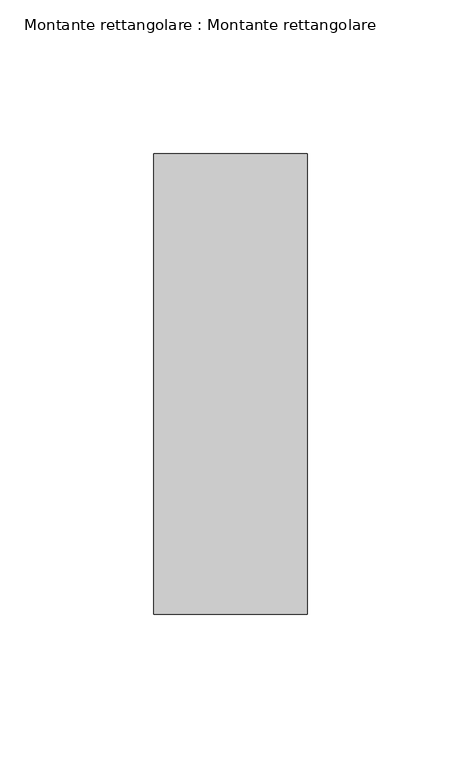
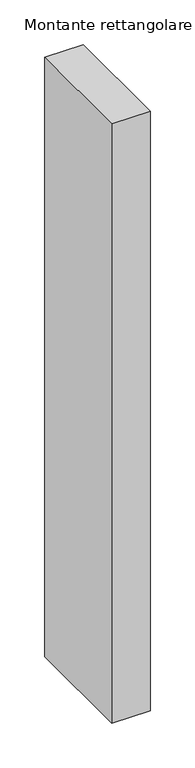
"""IFC4 building model written with IfcOpenShell, lengths in millimetres: member geometry, Montante rettangolare : Montante rettangolare."""

from ifc_helpers import new_model, si_unit, frame, origin, place, context, project, spatial, polyline, outline, extrude, source, transform, mapped, element, save


def montante_rettangolare_montante_rettangolare_07c532ff(model_context):
    return source(origin(), model_context, "Body", "SweptSolid", [
        extrude(outline(polyline([(0.0, 75.0), (0.0, -75.0), (-50.0, -75.0), (-50.0, 75.0), (0.0, 75.0)])), frame((0.0, 0.0, -820.0), z_axis=(0.0, 0.0, 1.0), x_axis=(1.0, 0.0, 0.0)), (0.0, 0.0, 1.0), 820.0),
    ])


if __name__ == "__main__":
    model = new_model("IFC4")
    model_context = context("Model", 3, world=origin())
    ifc_project = project(units=[si_unit("LENGTHUNIT", "METRE", prefix="MILLI")], contexts=[model_context])
    site = spatial("IfcSite", under=ifc_project)
    building = spatial("IfcBuilding", under=site)
    placement = place(None, origin())
    montante_rettangolare_montante_rettangolare_shape = montante_rettangolare_montante_rettangolare_07c532ff(model_context)
    element("IfcMember", 1, ObjectType="Montante rettangolare : Montante rettangolare", at=placement, inside=building, context=model_context, shape_type="MappedRepresentation", body=[
        mapped(montante_rettangolare_montante_rettangolare_shape, transform((0.0, 0.0, 0.0), x_axis=(1.0, 0.0, 0.0), y_axis=(0.0, 1.0, 0.0), z_axis=(0.0, 0.0, 1.0))),
    ])
    save(model, "model.ifc")

# Revit data of these elements
# Type "Montante rettangolare : Montante rettangolare"
#   built-in parameter 1007304 = 0.492126 (stored number, unit not read)
#   built-in parameter 1007301 = 0.082021 (stored number, unit not read)
#   built-in parameter 1007300 = 0.082021 (stored number, unit not read)
# Element 1 (IfcMember, "Montante rettangolare : Montante rettangolare")
#   Materials on its faces: "Acciaio"
# Materials
#   "Acciaio": class "Metallo", colour RGB 247 247 247, transparency 0, Description = "Acciaio, finitura zigrinata", Cost = 0
